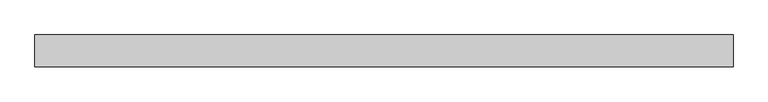
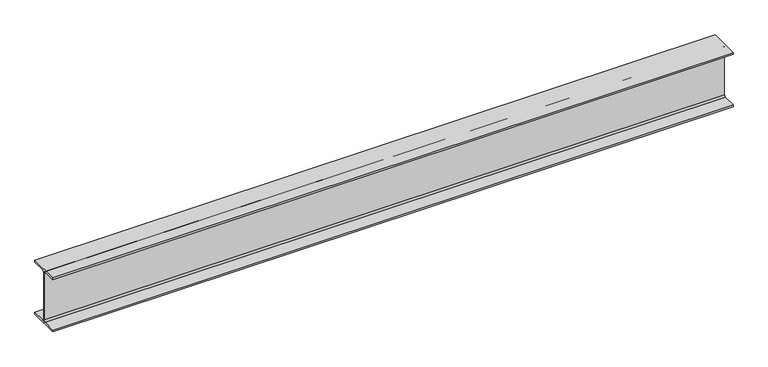
"""IFC4 building model written with IfcOpenShell, lengths in millimetres: beam geometry, Old_Steel Beam_H-KSD3502 : H_SB_ASB_H-250×125x6x9."""

import ifcopenshell
import ifcopenshell.guid

model = None  # the IFC model being written
_history = None  # IfcOwnerHistory: only IFC2X3 demands one
_inside = {}  # id of a spatial element -> (the spatial element, [elements in it])
_under = {}  # id of a project, library or spatial element -> (it, [spatial elements below it])
_declared = {}  # id of a project -> (the project, [libraries it declares])
_typed = {}  # id of a type object -> (the type object, [elements of that type])
_made_of = {}  # id of a material, layer set ... -> (it, [elements and type objects made of it])


def new_model(schema):
    """Start an empty IFC model of exactly this schema.

    Asked for "IFC4X3", IfcOpenShell would pick the latest addendum, in which some entities
    have other attributes; the version numbers below select the first issue.
    IFC2X3 requires an IfcOwnerHistory on every rooted entity: one is made here for all.
    """
    global model, _history
    if schema == "IFC4X3":
        model = ifcopenshell.file(schema_version=(4, 3, 0, 0))
    else:
        model = ifcopenshell.file(schema=schema)
    _inside.clear()
    _under.clear()
    _declared.clear()
    _typed.clear()
    _made_of.clear()
    _history = None
    if model.schema == "IFC2X3":
        org = make("IfcOrganization", Name="unknown")
        user = make(
            "IfcPersonAndOrganization",
            ThePerson=make("IfcPerson", FamilyName="unknown"),
            TheOrganization=org,
        )
        app = make(
            "IfcApplication",
            ApplicationDeveloper=org,
            Version="unknown",
            ApplicationFullName="unknown",
            ApplicationIdentifier="unknown",
        )
        _history = make(
            "IfcOwnerHistory",
            OwningUser=user,
            OwningApplication=app,
            ChangeAction="ADDED",
            CreationDate=0,
        )
    return model


def make(cls, **values):
    """One entity of the class cls with the attributes given. An attribute that is None is left unset."""
    return model.create_entity(
        cls, **{name: value for name, value in values.items() if value is not None}
    )


def rooted(cls, **values):
    """An entity with a GlobalId (a new one), such as an element, a storey or a relation."""
    return make(cls, GlobalId=ifcopenshell.guid.new(), OwnerHistory=_history, **values)


def si_unit(unit_type, name, prefix=None):
    """IfcSIUnit, for example si_unit("LENGTHUNIT", "METRE", prefix="MILLI")."""
    return make("IfcSIUnit", UnitType=unit_type, Prefix=prefix, Name=name)


def assignment(units):
    """IfcUnitAssignment: the units of a project."""
    return None if units is None else make("IfcUnitAssignment", Units=units)


def point(xyz):
    """IfcCartesianPoint."""
    return None if xyz is None else make("IfcCartesianPoint", Coordinates=xyz)


def direction(xyz):
    """IfcDirection."""
    return None if xyz is None else make("IfcDirection", DirectionRatios=xyz)


def frame(location, z_axis=None, x_axis=None):
    """IfcAxis2Placement3D, a coordinate frame: its origin and axes. An axis left out is left unset."""
    return make(
        "IfcAxis2Placement3D",
        Location=point(location),
        Axis=direction(z_axis),
        RefDirection=direction(x_axis),
    )


def frame_2d(location, x_axis=None):
    """IfcAxis2Placement2D, a coordinate frame in the plane: its origin and x axis."""
    return make(
        "IfcAxis2Placement2D", Location=point(location), RefDirection=direction(x_axis)
    )


def origin():
    """The frame at (0, 0, 0) with its axes left unset."""
    return frame((0.0, 0.0, 0.0))


def place(relative_to, where):
    """IfcLocalPlacement: puts the frame where relative to a parent placement (None: the world)."""
    return make(
        "IfcLocalPlacement", PlacementRelTo=relative_to, RelativePlacement=where
    )


def context(
    kind, dimensions, precision=None, world=None, true_north=None, identifier=None
):
    """IfcGeometricRepresentationContext, for example the 3D "Model" context."""
    return make(
        "IfcGeometricRepresentationContext",
        ContextIdentifier=identifier,
        ContextType=kind,
        CoordinateSpaceDimension=dimensions,
        Precision=precision,
        WorldCoordinateSystem=world,
        TrueNorth=true_north,
    )


def project(units=None, contexts=None):
    """IfcProject with its units and contexts."""
    return rooted(
        "IfcProject",
        Name="project",
        RepresentationContexts=contexts,
        UnitsInContext=assignment(units),
    )


def spatial(cls, under=None, at=None, **own):
    """A site, building, storey or space (cls), placed at a placement, below another one or the project."""
    s = rooted(cls, ObjectPlacement=at, **own)
    if under is not None:
        _under.setdefault(under.id(), (under, []))[1].append(s)
    return s


def polyline(points):
    """IfcPolyline through the points."""
    return make("IfcPolyline", Points=[point(p) for p in points])


def circle_curve(where, radius):
    """IfcCircle in the frame where."""
    return make("IfcCircle", Position=where, Radius=radius)


def trimmed(basis, trim1, trim2, sense, master):
    """IfcTrimmedCurve: the piece of a basis curve between two trims."""
    return make(
        "IfcTrimmedCurve",
        BasisCurve=basis,
        Trim1=trim1,
        Trim2=trim2,
        SenseAgreement=sense,
        MasterRepresentation=master,
    )


def segment(curve, same_sense, transition):
    """IfcCompositeCurveSegment."""
    return make(
        "IfcCompositeCurveSegment",
        Transition=transition,
        SameSense=same_sense,
        ParentCurve=curve,
    )


def composite_curve(segments, self_intersect=None):
    """IfcCompositeCurve: segments joined end to end."""
    return make("IfcCompositeCurve", Segments=segments, SelfIntersect=self_intersect)


def outline(outer, holes=None, kind="AREA"):
    """IfcArbitraryClosedProfileDef: a profile drawn as a closed curve; with holes, ...WithVoids."""
    if holes is None:
        return make("IfcArbitraryClosedProfileDef", ProfileType=kind, OuterCurve=outer)
    return make(
        "IfcArbitraryProfileDefWithVoids",
        ProfileType=kind,
        OuterCurve=outer,
        InnerCurves=holes,
    )


def extrude(swept, where, along, depth):
    """IfcExtrudedAreaSolid: the profile swept, set in the frame where, extruded along a direction by depth."""
    return make(
        "IfcExtrudedAreaSolid",
        SweptArea=swept,
        Position=where,
        ExtrudedDirection=direction(along),
        Depth=depth,
    )


def shape(context_of_items, identifier, shape_type, items):
    """IfcShapeRepresentation: the items that make up one representation, for example the "Body"."""
    return make(
        "IfcShapeRepresentation",
        ContextOfItems=context_of_items,
        RepresentationIdentifier=identifier,
        RepresentationType=shape_type,
        Items=items,
    )


def source(mapping_origin, context_of_items, identifier, shape_type, items):
    """IfcRepresentationMap: a shape defined once, which mapped items show again and again."""
    return make(
        "IfcRepresentationMap",
        MappingOrigin=mapping_origin,
        MappedRepresentation=shape(context_of_items, identifier, shape_type, items),
    )


def transform(
    local_origin,
    x_axis=None,
    y_axis=None,
    z_axis=None,
    scale=None,
    scale2=None,
    scale3=None,
    uniform=True,
):
    """IfcCartesianTransformationOperator3D, or its non-uniform kind. x_axis, y_axis, z_axis: its Axis1, 2, 3."""
    if uniform:
        return make(
            "IfcCartesianTransformationOperator3D",
            Axis1=direction(x_axis),
            Axis2=direction(y_axis),
            LocalOrigin=point(local_origin),
            Scale=scale,
            Axis3=direction(z_axis),
        )
    return make(
        "IfcCartesianTransformationOperator3DnonUniform",
        Axis1=direction(x_axis),
        Axis2=direction(y_axis),
        LocalOrigin=point(local_origin),
        Scale=scale,
        Axis3=direction(z_axis),
        Scale2=scale2,
        Scale3=scale3,
    )


def mapped(mapping_source, mapping_target):
    """IfcMappedItem: shows the shape of a source again, moved by a transform."""
    return make(
        "IfcMappedItem", MappingSource=mapping_source, MappingTarget=mapping_target
    )


def made_of(thing, what):
    """Note that an element or type object is made of a material, layer set ...; save() writes the relation."""
    if what is not None:
        _made_of.setdefault(what.id(), (what, []))[1].append(thing)
    return thing


def element(
    cls,
    number,
    at=None,
    inside=None,
    cuts=None,
    type_object=None,
    material=None,
    context=None,
    identifier="Body",
    shape_type=None,
    held_by="IfcProductDefinitionShape",
    body=None,
    shapes=None,
    **own,
):
    """One element of the class cls, such as IfcWall. Its Tag is "e" and its number.

    at: its placement. inside: the storey or other place that contains it. cuts: it is an
    opening in that element (IfcRelVoidsElement). A single representation is given by context,
    identifier, shape_type and body (its items); several are given by shapes. held_by: the class
    of the entity that holds the representations. save() writes the other relations.
    """
    e = rooted(cls, Tag="e%d" % number, ObjectPlacement=at, **own)
    if body is not None:
        shapes = [shape(context, identifier, shape_type, body)]
    if shapes is not None:
        e.Representation = make(held_by, Representations=shapes)
    if inside is not None:
        _inside.setdefault(inside.id(), (inside, []))[1].append(e)
    if cuts is not None:
        rooted(
            "IfcRelVoidsElement", RelatingBuildingElement=cuts, RelatedOpeningElement=e
        )
    if type_object is not None:
        _typed.setdefault(type_object.id(), (type_object, []))[1].append(e)
    return made_of(e, material)


def aggregate(whole, parts):
    """IfcRelAggregates: a whole, such as a stair, and the parts it consists of."""
    return rooted("IfcRelAggregates", RelatingObject=whole, RelatedObjects=parts)


def save(model, path):
    """Write the relations noted so far, then the file.

    IfcRelAggregates (storeys below a building ...), IfcRelContainedInSpatialStructure (elements
    in a storey), IfcRelDefinesByType, IfcRelAssociatesMaterial and IfcRelDeclares: one each for
    every whole, place, type object, material and project.
    """
    for whole, parts in _under.values():
        aggregate(whole, parts)
    for where, things in _inside.values():
        rooted(
            "IfcRelContainedInSpatialStructure",
            RelatedElements=things,
            RelatingStructure=where,
        )
    for kind, things in _typed.values():
        rooted("IfcRelDefinesByType", RelatedObjects=things, RelatingType=kind)
    for what, things in _made_of.values():
        rooted("IfcRelAssociatesMaterial", RelatedObjects=things, RelatingMaterial=what)
    for by, libraries in _declared.values():
        rooted("IfcRelDeclares", RelatingContext=by, RelatedDefinitions=libraries)
    model.write(path)


def beam_e590c642(model_context):
    return source(origin(), model_context, "Body", "SweptSolid", [
        extrude(outline(composite_curve([segment(polyline([(82.5, -141.5), (82.5, -151.7), (-82.5, -151.7), (-82.5, -141.5), (-11.9, -141.5)]), True, "CONTINUOUS"), segment(trimmed(circle_curve(frame_2d((-11.9, -132.6)), 8.9), [point((-11.9, -141.5))], [point((-3.0, -132.6))], True, "CARTESIAN"), True, "CONTINUOUS"), segment(polyline([(-3.0, -132.6), (-3.0, 132.6)]), True, "CONTINUOUS"), segment(trimmed(circle_curve(frame_2d((-11.9, 132.6)), 8.9), [point((-3.0, 132.6))], [point((-11.9, 141.5))], True, "CARTESIAN"), True, "CONTINUOUS"), segment(polyline([(-11.9, 141.5), (-82.5, 141.5), (-82.5, 151.7), (82.5, 151.7), (82.5, 141.5), (11.9, 141.5)]), True, "CONTINUOUS"), segment(trimmed(circle_curve(frame_2d((11.9, 132.6)), 8.9), [point((11.9, 141.5))], [point((3.0, 132.6))], True, "CARTESIAN"), True, "CONTINUOUS"), segment(polyline([(3.0, 132.6), (3.0, -132.6)]), True, "CONTINUOUS"), segment(trimmed(circle_curve(frame_2d((11.9, -132.6)), 8.9), [point((3.0, -132.6))], [point((11.9, -141.5))], True, "CARTESIAN"), True, "CONTINUOUS"), segment(polyline([(11.9, -141.5), (82.5, -141.5)]), True, "CONTINUOUS")], self_intersect=False)), frame((-1718.3833333, 0.0, 0.0), z_axis=(1.0, 0.0, 0.0), x_axis=(0.0, 1.0, 0.0)), (0.0, 0.0, 1.0), 3623.1833333),
    ])


if __name__ == "__main__":
    model = new_model("IFC4")
    model_context = context("Model", 3, world=origin())
    ifc_project = project(units=[si_unit("LENGTHUNIT", "METRE", prefix="MILLI")], contexts=[model_context])
    site = spatial("IfcSite", under=ifc_project)
    building = spatial("IfcBuilding", under=site)
    placement = place(None, origin())
    beam_shape = beam_e590c642(model_context)
    element("IfcBeam", 1, ObjectType="Old_Steel Beam_H-KSD3502 : H_SB_ASB_H-250×125x6x9", at=placement, inside=building, context=model_context, shape_type="MappedRepresentation", body=[
        mapped(beam_shape, transform((0.0, 0.0, 0.0), x_axis=(1.0, 0.0, 0.0), y_axis=(0.0, 1.0, 0.0), z_axis=(0.0, 0.0, 1.0))),
    ])
    save(model, "model.ifc")

# Revit data of these elements
# Type "Old_Steel Beam_H-KSD3502 : H_SB_ASB_H-250×125x6x9"
#   Width = 12.5 cm
#   Web Thickness = 0.6 cm
#   Web Fillet = 1.2 cm
#   Warping Constant = 42539.8 cm⁶
#   Torsional Moment of Inertia = 7.8102 cm⁴
#   Torsional Modulus = 1.0 cm³
#   Section Area = 37.66 cm²
#   Plastic Modulus weak axis = 73.1 cm³
#   Plastic Modulus strong axis = 366.0 cm³
#   Perimeter = 0.97 m²/m
#   Nominal Weight = 29.60 kgf/m
#   Moment of Inertia weak axis = 294.00 cm⁴
#   Moment of Inertia strong axis = 4050.00 cm⁴
#   Height = 25.0 cm
#   Flange Thickness = 0.9 cm
#   Elastic Modulus weak axis = 47.0 cm³
#   Elastic Modulus strong axis = 324.0 cm³
#   Centroid Vertical = 12.5 cm
#   Centroid Horizontal = 6.25 cm
#   Length [instance default] = 1.5240 m
#   Structural Material [instance default] = Steel, 45-345
#   Assembly Code = ""
# Element 1 (IfcBeam, "Old_Steel Beam_H-KSD3502 : H_SB_ASB_H-250×125x6x9")
#   Structural Material = none
# Materials
#   "Steel, 45-345": class "Metal", colour RGB 189 187 185, transparency 0, Description = "Steel 345 MPa", Cost = 0
